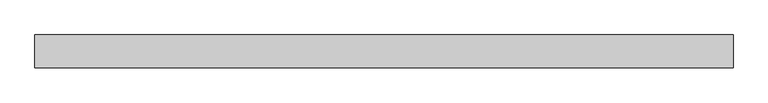
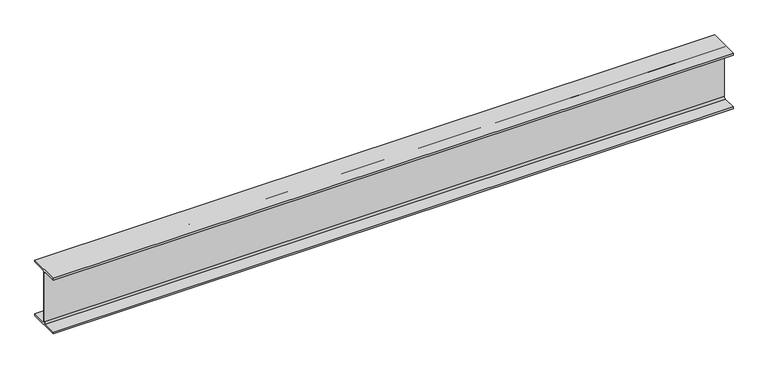
"""IFC4 building model written with IfcOpenShell, lengths in millimetres: beam geometry, Old_Steel Beam_H-KSD3502 : H_SB_ASB_H-200×200x8x12."""

import ifcopenshell
import ifcopenshell.guid

model = None  # the IFC model being written
_history = None  # IfcOwnerHistory: only IFC2X3 demands one
_inside = {}  # id of a spatial element -> (the spatial element, [elements in it])
_under = {}  # id of a project, library or spatial element -> (it, [spatial elements below it])
_declared = {}  # id of a project -> (the project, [libraries it declares])
_typed = {}  # id of a type object -> (the type object, [elements of that type])
_made_of = {}  # id of a material, layer set ... -> (it, [elements and type objects made of it])


def new_model(schema):
    """Start an empty IFC model of exactly this schema.

    Asked for "IFC4X3", IfcOpenShell would pick the latest addendum, in which some entities
    have other attributes; the version numbers below select the first issue.
    IFC2X3 requires an IfcOwnerHistory on every rooted entity: one is made here for all.
    """
    global model, _history
    if schema == "IFC4X3":
        model = ifcopenshell.file(schema_version=(4, 3, 0, 0))
    else:
        model = ifcopenshell.file(schema=schema)
    _inside.clear()
    _under.clear()
    _declared.clear()
    _typed.clear()
    _made_of.clear()
    _history = None
    if model.schema == "IFC2X3":
        org = make("IfcOrganization", Name="unknown")
        user = make(
            "IfcPersonAndOrganization",
            ThePerson=make("IfcPerson", FamilyName="unknown"),
            TheOrganization=org,
        )
        app = make(
            "IfcApplication",
            ApplicationDeveloper=org,
            Version="unknown",
            ApplicationFullName="unknown",
            ApplicationIdentifier="unknown",
        )
        _history = make(
            "IfcOwnerHistory",
            OwningUser=user,
            OwningApplication=app,
            ChangeAction="ADDED",
            CreationDate=0,
        )
    return model


def make(cls, **values):
    """One entity of the class cls with the attributes given. An attribute that is None is left unset."""
    return model.create_entity(
        cls, **{name: value for name, value in values.items() if value is not None}
    )


def rooted(cls, **values):
    """An entity with a GlobalId (a new one), such as an element, a storey or a relation."""
    return make(cls, GlobalId=ifcopenshell.guid.new(), OwnerHistory=_history, **values)


def si_unit(unit_type, name, prefix=None):
    """IfcSIUnit, for example si_unit("LENGTHUNIT", "METRE", prefix="MILLI")."""
    return make("IfcSIUnit", UnitType=unit_type, Prefix=prefix, Name=name)


def assignment(units):
    """IfcUnitAssignment: the units of a project."""
    return None if units is None else make("IfcUnitAssignment", Units=units)


def point(xyz):
    """IfcCartesianPoint."""
    return None if xyz is None else make("IfcCartesianPoint", Coordinates=xyz)


def direction(xyz):
    """IfcDirection."""
    return None if xyz is None else make("IfcDirection", DirectionRatios=xyz)


def frame(location, z_axis=None, x_axis=None):
    """IfcAxis2Placement3D, a coordinate frame: its origin and axes. An axis left out is left unset."""
    return make(
        "IfcAxis2Placement3D",
        Location=point(location),
        Axis=direction(z_axis),
        RefDirection=direction(x_axis),
    )


def frame_2d(location, x_axis=None):
    """IfcAxis2Placement2D, a coordinate frame in the plane: its origin and x axis."""
    return make(
        "IfcAxis2Placement2D", Location=point(location), RefDirection=direction(x_axis)
    )


def origin():
    """The frame at (0, 0, 0) with its axes left unset."""
    return frame((0.0, 0.0, 0.0))


def place(relative_to, where):
    """IfcLocalPlacement: puts the frame where relative to a parent placement (None: the world)."""
    return make(
        "IfcLocalPlacement", PlacementRelTo=relative_to, RelativePlacement=where
    )


def context(
    kind, dimensions, precision=None, world=None, true_north=None, identifier=None
):
    """IfcGeometricRepresentationContext, for example the 3D "Model" context."""
    return make(
        "IfcGeometricRepresentationContext",
        ContextIdentifier=identifier,
        ContextType=kind,
        CoordinateSpaceDimension=dimensions,
        Precision=precision,
        WorldCoordinateSystem=world,
        TrueNorth=true_north,
    )


def project(units=None, contexts=None):
    """IfcProject with its units and contexts."""
    return rooted(
        "IfcProject",
        Name="project",
        RepresentationContexts=contexts,
        UnitsInContext=assignment(units),
    )


def spatial(cls, under=None, at=None, **own):
    """A site, building, storey or space (cls), placed at a placement, below another one or the project."""
    s = rooted(cls, ObjectPlacement=at, **own)
    if under is not None:
        _under.setdefault(under.id(), (under, []))[1].append(s)
    return s


def polyline(points):
    """IfcPolyline through the points."""
    return make("IfcPolyline", Points=[point(p) for p in points])


def circle_curve(where, radius):
    """IfcCircle in the frame where."""
    return make("IfcCircle", Position=where, Radius=radius)


def trimmed(basis, trim1, trim2, sense, master):
    """IfcTrimmedCurve: the piece of a basis curve between two trims."""
    return make(
        "IfcTrimmedCurve",
        BasisCurve=basis,
        Trim1=trim1,
        Trim2=trim2,
        SenseAgreement=sense,
        MasterRepresentation=master,
    )


def segment(curve, same_sense, transition):
    """IfcCompositeCurveSegment."""
    return make(
        "IfcCompositeCurveSegment",
        Transition=transition,
        SameSense=same_sense,
        ParentCurve=curve,
    )


def composite_curve(segments, self_intersect=None):
    """IfcCompositeCurve: segments joined end to end."""
    return make("IfcCompositeCurve", Segments=segments, SelfIntersect=self_intersect)


def outline(outer, holes=None, kind="AREA"):
    """IfcArbitraryClosedProfileDef: a profile drawn as a closed curve; with holes, ...WithVoids."""
    if holes is None:
        return make("IfcArbitraryClosedProfileDef", ProfileType=kind, OuterCurve=outer)
    return make(
        "IfcArbitraryProfileDefWithVoids",
        ProfileType=kind,
        OuterCurve=outer,
        InnerCurves=holes,
    )


def extrude(swept, where, along, depth):
    """IfcExtrudedAreaSolid: the profile swept, set in the frame where, extruded along a direction by depth."""
    return make(
        "IfcExtrudedAreaSolid",
        SweptArea=swept,
        Position=where,
        ExtrudedDirection=direction(along),
        Depth=depth,
    )


def shape(context_of_items, identifier, shape_type, items):
    """IfcShapeRepresentation: the items that make up one representation, for example the "Body"."""
    return make(
        "IfcShapeRepresentation",
        ContextOfItems=context_of_items,
        RepresentationIdentifier=identifier,
        RepresentationType=shape_type,
        Items=items,
    )


def source(mapping_origin, context_of_items, identifier, shape_type, items):
    """IfcRepresentationMap: a shape defined once, which mapped items show again and again."""
    return make(
        "IfcRepresentationMap",
        MappingOrigin=mapping_origin,
        MappedRepresentation=shape(context_of_items, identifier, shape_type, items),
    )


def transform(
    local_origin,
    x_axis=None,
    y_axis=None,
    z_axis=None,
    scale=None,
    scale2=None,
    scale3=None,
    uniform=True,
):
    """IfcCartesianTransformationOperator3D, or its non-uniform kind. x_axis, y_axis, z_axis: its Axis1, 2, 3."""
    if uniform:
        return make(
            "IfcCartesianTransformationOperator3D",
            Axis1=direction(x_axis),
            Axis2=direction(y_axis),
            LocalOrigin=point(local_origin),
            Scale=scale,
            Axis3=direction(z_axis),
        )
    return make(
        "IfcCartesianTransformationOperator3DnonUniform",
        Axis1=direction(x_axis),
        Axis2=direction(y_axis),
        LocalOrigin=point(local_origin),
        Scale=scale,
        Axis3=direction(z_axis),
        Scale2=scale2,
        Scale3=scale3,
    )


def mapped(mapping_source, mapping_target):
    """IfcMappedItem: shows the shape of a source again, moved by a transform."""
    return make(
        "IfcMappedItem", MappingSource=mapping_source, MappingTarget=mapping_target
    )


def made_of(thing, what):
    """Note that an element or type object is made of a material, layer set ...; save() writes the relation."""
    if what is not None:
        _made_of.setdefault(what.id(), (what, []))[1].append(thing)
    return thing


def element(
    cls,
    number,
    at=None,
    inside=None,
    cuts=None,
    type_object=None,
    material=None,
    context=None,
    identifier="Body",
    shape_type=None,
    held_by="IfcProductDefinitionShape",
    body=None,
    shapes=None,
    **own,
):
    """One element of the class cls, such as IfcWall. Its Tag is "e" and its number.

    at: its placement. inside: the storey or other place that contains it. cuts: it is an
    opening in that element (IfcRelVoidsElement). A single representation is given by context,
    identifier, shape_type and body (its items); several are given by shapes. held_by: the class
    of the entity that holds the representations. save() writes the other relations.
    """
    e = rooted(cls, Tag="e%d" % number, ObjectPlacement=at, **own)
    if body is not None:
        shapes = [shape(context, identifier, shape_type, body)]
    if shapes is not None:
        e.Representation = make(held_by, Representations=shapes)
    if inside is not None:
        _inside.setdefault(inside.id(), (inside, []))[1].append(e)
    if cuts is not None:
        rooted(
            "IfcRelVoidsElement", RelatingBuildingElement=cuts, RelatedOpeningElement=e
        )
    if type_object is not None:
        _typed.setdefault(type_object.id(), (type_object, []))[1].append(e)
    return made_of(e, material)


def aggregate(whole, parts):
    """IfcRelAggregates: a whole, such as a stair, and the parts it consists of."""
    return rooted("IfcRelAggregates", RelatingObject=whole, RelatedObjects=parts)


def save(model, path):
    """Write the relations noted so far, then the file.

    IfcRelAggregates (storeys below a building ...), IfcRelContainedInSpatialStructure (elements
    in a storey), IfcRelDefinesByType, IfcRelAssociatesMaterial and IfcRelDeclares: one each for
    every whole, place, type object, material and project.
    """
    for whole, parts in _under.values():
        aggregate(whole, parts)
    for where, things in _inside.values():
        rooted(
            "IfcRelContainedInSpatialStructure",
            RelatedElements=things,
            RelatingStructure=where,
        )
    for kind, things in _typed.values():
        rooted("IfcRelDefinesByType", RelatedObjects=things, RelatingType=kind)
    for what, things in _made_of.values():
        rooted("IfcRelAssociatesMaterial", RelatedObjects=things, RelatingMaterial=what)
    for by, libraries in _declared.values():
        rooted("IfcRelDeclares", RelatingContext=by, RelatedDefinitions=libraries)
    model.write(path)


def beam_fe681a5f(model_context):
    return source(origin(), model_context, "Body", "SweptSolid", [
        extrude(outline(composite_curve([segment(polyline([(82.5, -141.5), (82.5, -151.7), (-82.5, -151.7), (-82.5, -141.5), (-11.9, -141.5)]), True, "CONTINUOUS"), segment(trimmed(circle_curve(frame_2d((-11.9, -132.6)), 8.9), [point((-11.9, -141.5))], [point((-3.0, -132.6))], True, "CARTESIAN"), True, "CONTINUOUS"), segment(polyline([(-3.0, -132.6), (-3.0, 132.6)]), True, "CONTINUOUS"), segment(trimmed(circle_curve(frame_2d((-11.9, 132.6)), 8.9), [point((-3.0, 132.6))], [point((-11.9, 141.5))], True, "CARTESIAN"), True, "CONTINUOUS"), segment(polyline([(-11.9, 141.5), (-82.5, 141.5), (-82.5, 151.7), (82.5, 151.7), (82.5, 141.5), (11.9, 141.5)]), True, "CONTINUOUS"), segment(trimmed(circle_curve(frame_2d((11.9, 132.6)), 8.9), [point((11.9, 141.5))], [point((3.0, 132.6))], True, "CARTESIAN"), True, "CONTINUOUS"), segment(polyline([(3.0, 132.6), (3.0, -132.6)]), True, "CONTINUOUS"), segment(trimmed(circle_curve(frame_2d((11.9, -132.6)), 8.9), [point((3.0, -132.6))], [point((11.9, -141.5))], True, "CARTESIAN"), True, "CONTINUOUS"), segment(polyline([(11.9, -141.5), (82.5, -141.5)]), True, "CONTINUOUS")], self_intersect=False)), frame((-1805.839182, 0.0, 0.0), z_axis=(1.0, 0.0, 0.0), x_axis=(0.0, 1.0, 0.0)), (0.0, 0.0, 1.0), 3511.0476207),
    ])


if __name__ == "__main__":
    model = new_model("IFC4")
    model_context = context("Model", 3, world=origin())
    ifc_project = project(units=[si_unit("LENGTHUNIT", "METRE", prefix="MILLI")], contexts=[model_context])
    site = spatial("IfcSite", under=ifc_project)
    building = spatial("IfcBuilding", under=site)
    placement = place(None, origin())
    beam_shape = beam_fe681a5f(model_context)
    element("IfcBeam", 1, ObjectType="Old_Steel Beam_H-KSD3502 : H_SB_ASB_H-200×200x8x12", at=placement, inside=building, context=model_context, shape_type="MappedRepresentation", body=[
        mapped(beam_shape, transform((0.0, 0.0, 0.0), x_axis=(1.0, 0.0, 0.0), y_axis=(0.0, 1.0, 0.0), z_axis=(0.0, 0.0, 1.0))),
    ])
    save(model, "model.ifc")

# Revit data of these elements
# Type "Old_Steel Beam_H-KSD3502 : H_SB_ASB_H-200×200x8x12"
#   Width = 20.0 cm
#   Web Thickness = 0.8 cm
#   Web Fillet = 1.3 cm
#   Warping Constant = 141376.0 cm⁶
#   Torsional Moment of Inertia = 26.2485 cm⁴
#   Torsional Modulus = 1.0 cm³
#   Section Area = 63.53 cm²
#   Plastic Modulus weak axis = 244.0 cm³
#   Plastic Modulus strong axis = 525.0 cm³
#   Perimeter = 1.16 m²/m
#   Nominal Weight = 49.90 kgf/m
#   Moment of Inertia weak axis = 1600.00 cm⁴
#   Moment of Inertia strong axis = 4720.00 cm⁴
#   Height = 20.0 cm
#   Flange Thickness = 1.2 cm
#   Elastic Modulus weak axis = 160.0 cm³
#   Elastic Modulus strong axis = 472.0 cm³
#   Centroid Vertical = 10.0 cm
#   Centroid Horizontal = 10.0 cm
#   Length [instance default] = 1.5240 m
#   Structural Material [instance default] = Steel, 45-345
#   Assembly Code = ""
# Element 1 (IfcBeam, "Old_Steel Beam_H-KSD3502 : H_SB_ASB_H-200×200x8x12")
#   Structural Material = none
# Materials
#   "Steel, 45-345": class "Metal", colour RGB 189 187 185, transparency 0, Description = "Steel 345 MPa", Cost = 0
